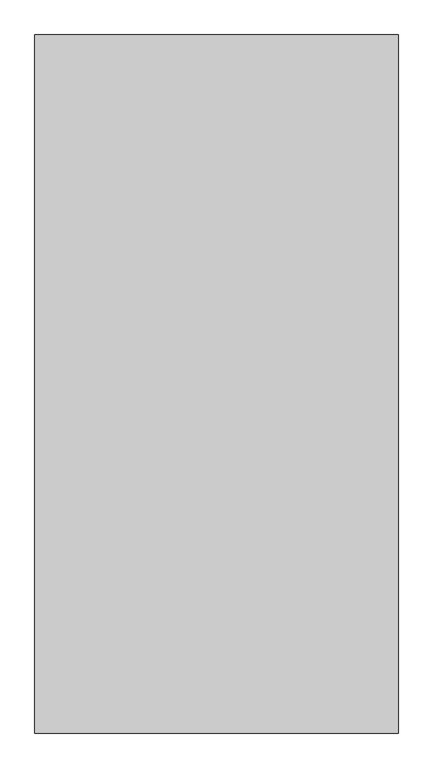
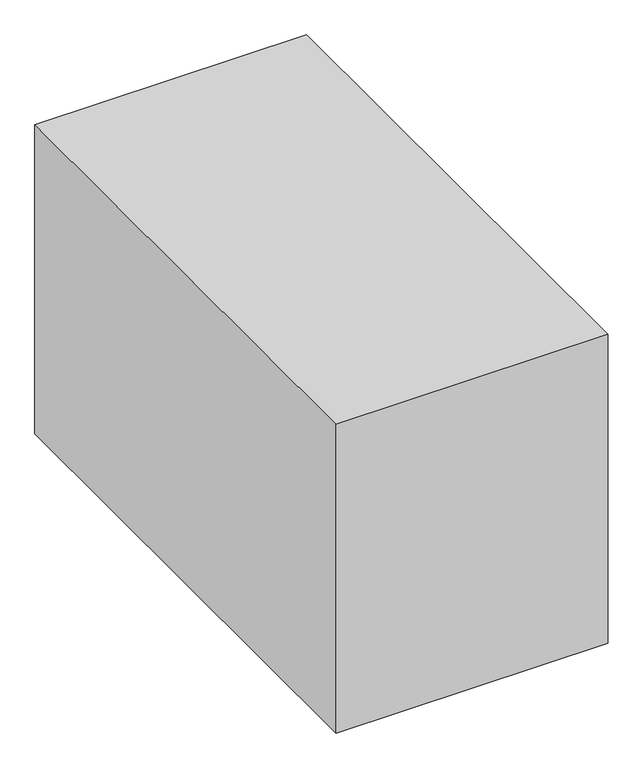
"""IFC4 building model written with IfcOpenShell, lengths in millimetres: proxy geometry, Space Planning Box_hec : Space Planning Box_hec."""

from ifc_helpers import new_model, si_unit, origin, origin_with_axes, place, context, project, spatial, polyline, outline, extrude, source, transform, mapped, element, save


def generic_models_7902148a(model_context):
    return source(origin(), model_context, "Body", "SweptSolid", [
        extrude(outline(polyline([(2500.0, 4800.0), (2500.0, -4800.0), (-2500.0, -4800.0), (-2500.0, 4800.0), (2500.0, 4800.0)])), origin_with_axes(), (0.0, 0.0, 1.0), 6000.0),
    ])


if __name__ == "__main__":
    model = new_model("IFC4")
    model_context = context("Model", 3, world=origin())
    ifc_project = project(units=[si_unit("LENGTHUNIT", "METRE", prefix="MILLI")], contexts=[model_context])
    site = spatial("IfcSite", under=ifc_project)
    building = spatial("IfcBuilding", under=site)
    placement = place(None, origin())
    generic_models_shape = generic_models_7902148a(model_context)
    element("IfcBuildingElementProxy", 1, Name="Space Planning Box_hec : Space Planning Box_hec", ObjectType="Space Planning Box_hec : Space Planning Box_hec", at=placement, inside=building, context=model_context, shape_type="MappedRepresentation", body=[
        mapped(generic_models_shape, transform((0.0, 0.0, 0.0), x_axis=(1.0, 0.0, 0.0), y_axis=(0.0, 1.0, 0.0), z_axis=(0.0, 0.0, 1.0))),
    ])
    save(model, "model.ifc")

# Revit data of these elements
# Type "Space Planning Box_hec : Space Planning Box_hec"
#   Type Comments = "..."
#   Room Name [instance default] = "?"
#   Interior Finish [instance default] = ""
#   Exterior Finish [instance default] = ""
#   Department [instance default] = ""
#   Assembly Code = "..."
#   Width [instance default] = 1524 mm
#   Program Area [instance default] = 0.00 m²
#   Length [instance default] = 1524 mm
#   Height [instance default] = 1524 mm
#   Area [instance default] = 2.32258 m²
#   Fill Color [instance default] = Cyan
#   Default Elevation = 0
# Element 1 (IfcBuildingElementProxy, "Space Planning Box_hec : Space Planning Box_hec")
#   Room Name = "Document Room"
#   Interior Finish = "IF2-1"
#   Exterior Finish = "EF1"
#   Department = "AR"
#   Width = 5000 mm
#   Program Area = 48.00 m²
#   Length = 9600 mm
#   Height = 6000 mm
#   Area = 48.00 m²
#   Materials on its faces: "Cyan"
# Materials
#   "Cyan": class "Generic", colour RGB 0 255 255, transparency 0.2, Cost = 0
